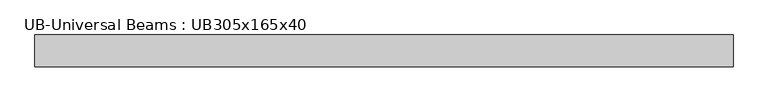
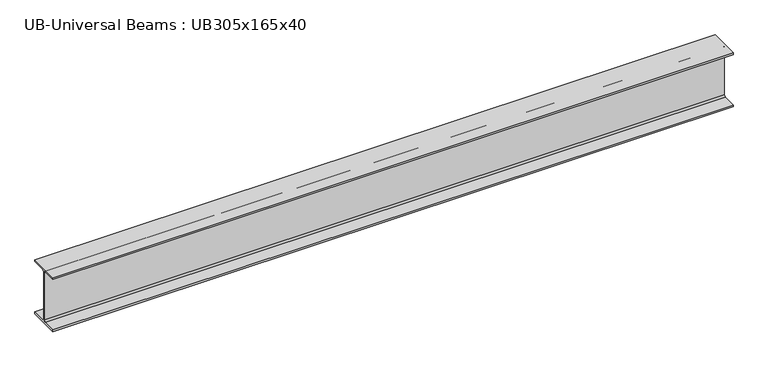
"""IFC4 building model written with IfcOpenShell, lengths in millimetres: beam geometry, UB-Universal Beams : UB305x165x40."""

from ifc_helpers import new_model, si_unit, point, frame, frame_2d, origin, place, context, project, spatial, polyline, circle_curve, trimmed, segment, composite_curve, outline, extrude, source, transform, mapped, element, save


def ub_universal_beams_ub305x165x40_c5b634f3(model_context):
    return source(origin(), model_context, "Body", "SweptSolid", [
        extrude(outline(composite_curve([segment(polyline([(82.5, -141.5), (82.5, -151.7), (-82.5, -151.7), (-82.5, -141.5), (-11.9, -141.5)]), True, "CONTINUOUS"), segment(trimmed(circle_curve(frame_2d((-11.9, -132.6)), 8.9), [point((-11.9, -141.5))], [point((-3.0, -132.6))], True, "CARTESIAN"), True, "CONTINUOUS"), segment(polyline([(-3.0, -132.6), (-3.0, 132.6)]), True, "CONTINUOUS"), segment(trimmed(circle_curve(frame_2d((-11.9, 132.6)), 8.9), [point((-3.0, 132.6))], [point((-11.9, 141.5))], True, "CARTESIAN"), True, "CONTINUOUS"), segment(polyline([(-11.9, 141.5), (-82.5, 141.5), (-82.5, 151.7), (82.5, 151.7), (82.5, 141.5), (11.9, 141.5)]), True, "CONTINUOUS"), segment(trimmed(circle_curve(frame_2d((11.9, 132.6)), 8.9), [point((11.9, 141.5))], [point((3.0, 132.6))], True, "CARTESIAN"), True, "CONTINUOUS"), segment(polyline([(3.0, 132.6), (3.0, -132.6)]), True, "CONTINUOUS"), segment(trimmed(circle_curve(frame_2d((11.9, -132.6)), 8.9), [point((3.0, -132.6))], [point((11.9, -141.5))], True, "CARTESIAN"), True, "CONTINUOUS"), segment(polyline([(11.9, -141.5), (82.5, -141.5)]), True, "CONTINUOUS")], self_intersect=False)), frame((-1802.75, 0.0, 0.0), z_axis=(1.0, 0.0, 0.0), x_axis=(0.0, 1.0, 0.0)), (0.0, 0.0, 1.0), 3605.5),
    ])


if __name__ == "__main__":
    model = new_model("IFC4")
    model_context = context("Model", 3, world=origin())
    ifc_project = project(units=[si_unit("LENGTHUNIT", "METRE", prefix="MILLI")], contexts=[model_context])
    site = spatial("IfcSite", under=ifc_project)
    building = spatial("IfcBuilding", under=site)
    placement = place(None, origin())
    ub_universal_beams_ub305x165x40_shape = ub_universal_beams_ub305x165x40_c5b634f3(model_context)
    element("IfcBeam", 1, ObjectType="UB-Universal Beams : UB305x165x40", at=placement, inside=building, context=model_context, shape_type="MappedRepresentation", body=[
        mapped(ub_universal_beams_ub305x165x40_shape, transform((0.0, 0.0, 0.0), x_axis=(1.0, 0.0, 0.0), y_axis=(0.0, 1.0, 0.0), z_axis=(0.0, 0.0, 1.0))),
    ])
    save(model, "model.ifc")

# Revit data of these elements
# Type "UB-Universal Beams : UB305x165x40"
#   Section Name Key = "UB305X165X40"
#   Width = 16.5 cm
#   Web Thickness = 0.6 cm
#   Web Fillet = 0.89 cm
#   Warping Constant = 164000.0 cm⁶
#   Torsional Moment of Inertia = 14.70 cm⁴
#   Section Area = 51.3 cm²
#   Plastic Modulus weak axis = 142.0 cm³
#   Plastic Modulus strong axis = 623.0 cm³
#   Nominal Weight = 40.2999 kgf/m
#   Moment of Inertia weak axis = 764.00 cm⁴
#   Moment of Inertia strong axis = 8503.00 cm⁴
#   Height = 30.34 cm
#   Flange Thickness = 1.02 cm
#   Elastic Modulus weak axis = 92.6 cm³
#   Elastic Modulus strong axis = 560.0 cm³
#   Centroid Vertical = 15.17 cm
#   Centroid Horizontal = 8.25 cm
#   Bolt Spacing = 9.0 cm
#   Length [instance default] = 1500 mm
#   Structural Material [instance default] = Metal - Steel 43-275
#   Type Comments = ""
#   Assembly Code = ""
# Element 1 (IfcBeam, "UB-Universal Beams : UB305x165x40")
#   Materials on its faces: "Metal - Steel 43-275"
# Materials
#   "Metal - Steel 43-275": class "Metal", colour RGB 247 247 247, transparency 0, Cost = 0
